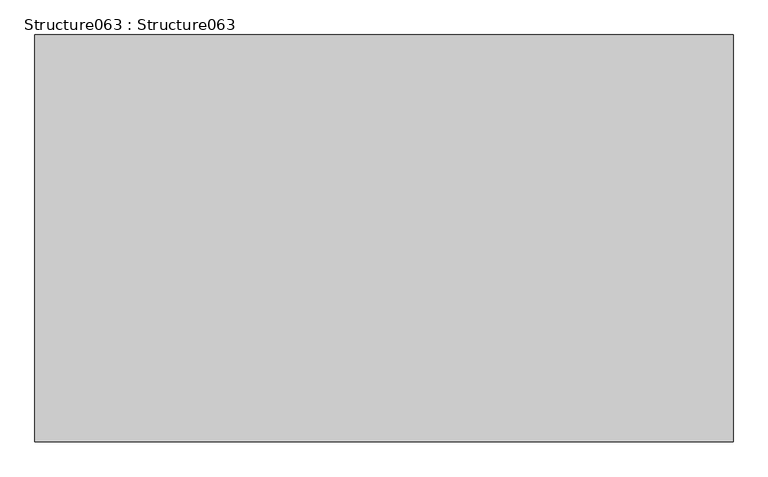
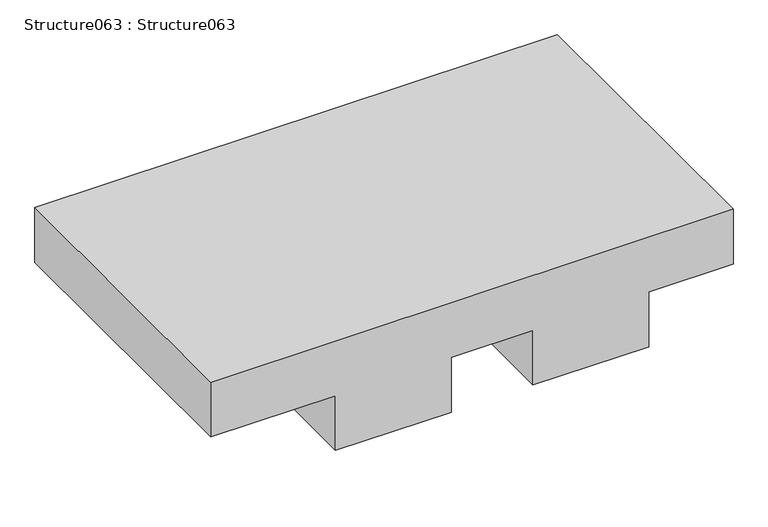
"""IFC4 building model written with IfcOpenShell, lengths in millimetres: proxy geometry, Structure063 : Structure063."""

from ifc_helpers import new_model, si_unit, frame, origin, place, context, project, spatial, polyline, outline, extrude, source, transform, mapped, element, save


def structure063_structure063_53ccb683(model_context):
    return source(origin(), model_context, "Body", "SweptSolid", [
        extrude(outline(polyline([(36150.296, 4850.5121633), (36150.296, 5669.8112048), (35769.296, 5669.8112048), (35769.296, 6431.8112048), (36150.296, 6431.8112048), (36150.296, 6968.3862048), (35769.296, 6968.3862048), (35769.296, 7730.3862048), (36150.296, 7730.3862048), (36150.296, 8283.3477835), (36531.296, 8283.3477835), (36531.296, 4850.5121633), (36150.296, 4850.5121633)])), frame((0.0, -3747.9491938, 0.0), z_axis=(0.0, 1.0, 0.0), x_axis=(0.0, 0.0, 1.0)), (0.0, 0.0, 1.0), 2000.0),
    ])


if __name__ == "__main__":
    model = new_model("IFC4")
    model_context = context("Model", 3, world=origin())
    ifc_project = project(units=[si_unit("LENGTHUNIT", "METRE", prefix="MILLI")], contexts=[model_context])
    site = spatial("IfcSite", under=ifc_project)
    building = spatial("IfcBuilding", under=site)
    placement = place(None, origin())
    structure063_structure063_shape = structure063_structure063_53ccb683(model_context)
    element("IfcBuildingElementProxy", 1, Name="Structure063 : Structure063", ObjectType="Structure063 : Structure063", at=placement, inside=building, context=model_context, shape_type="MappedRepresentation", body=[
        mapped(structure063_structure063_shape, transform((0.0, 0.0, 0.0), x_axis=(1.0, 0.0, 0.0), y_axis=(0.0, 1.0, 0.0), z_axis=(0.0, 0.0, 1.0))),
    ])
    save(model, "model.ifc")

# Revit data of these elements
# Type "Structure063 : Structure063"
#   NameOverride = "Structure063"
# Element 1 (IfcBuildingElementProxy, "Structure063 : Structure063")
#   Materials on its faces: "CONCRETE SLAB W/ GRADE BEAM (SEE STRUCT DWGS)"
# Materials
#   "CONCRETE SLAB W/ GRADE BEAM (SEE STRUCT DWGS)": class "Unassigned", colour RGB 128 128 128, transparency 0, Cost = 0
